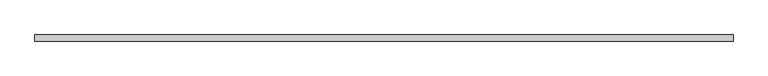
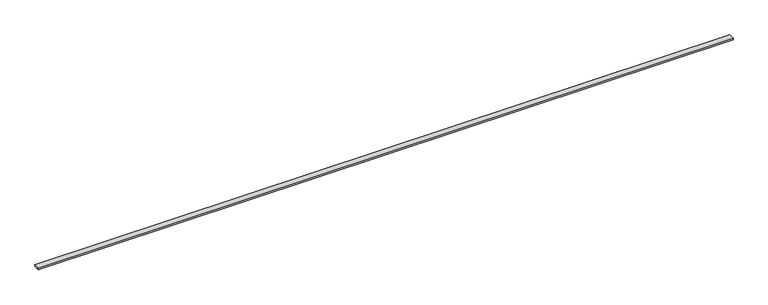
"""IFC4 building model written with IfcOpenShell, lengths in millimetres: proxy geometry, Generic Models 7:Generic Models 1:337419:Generic Models 1:337419 : Generic Models 7:Generic Models 1:337419:41 : Generic Models 7:Generic Models 1:337419:Generic Models 1:337419 : Generic Models 7:Generic Models 1:337419:301336."""

from ifc_helpers import new_model, si_unit, frame, origin, place, context, project, spatial, polyline, outline, extrude, source, transform, mapped, element, save


def generic_models_0fbd16a8(model_context):
    return source(origin(), model_context, "Body", "SweptSolid", [
        extrude(outline(polyline([(596182.8367242, -536511.1096233), (596182.8367242, -536554.1163841), (591306.0367242, -536554.1163841), (591306.0367242, -536511.1096233), (596182.8367242, -536511.1096233)])), frame((0.0, 0.0, 10085.5977062), z_axis=(0.0, 0.0, 1.0), x_axis=(1.0, 0.0, 0.0)), (0.0, 0.0, 1.0), 9.6384173),
    ])


if __name__ == "__main__":
    model = new_model("IFC4")
    model_context = context("Model", 3, world=origin())
    ifc_project = project(units=[si_unit("LENGTHUNIT", "METRE", prefix="MILLI")], contexts=[model_context])
    site = spatial("IfcSite", under=ifc_project)
    building = spatial("IfcBuilding", under=site)
    placement = place(None, origin())
    generic_models_shape = generic_models_0fbd16a8(model_context)
    element("IfcBuildingElementProxy", 1, Name="Generic Models 7:Generic Models 1:337419:Generic Models 1:337419 : Generic Models 7:Generic Models 1:337419:41 : Generic Models 7:Generic Models 1:337419:Generic Models 1:337419 : Generic Models 7:Generic Models 1:337419:301336", ObjectType="Generic Models 7:Generic Models 1:337419:Generic Models 1:337419 : Generic Models 7:Generic Models 1:337419:41 : Generic Models 7:Generic Models 1:337419:Generic Models 1:337419 : Generic Models 7:Generic Models 1:337419:301336", at=placement, inside=building, context=model_context, shape_type="MappedRepresentation", body=[
        mapped(generic_models_shape, transform((0.0, 0.0, 0.0), x_axis=(1.0, 0.0, 0.0), y_axis=(0.0, 1.0, 0.0), z_axis=(0.0, 0.0, 1.0))),
    ])
    save(model, "model.ifc")

# Revit data of these elements
# Type "Generic Models 7:Generic Models 1:337419:Generic Models 1:337419 : Generic Models 7:Generic Models 1:337419:41 : Generic Models 7:Generic Models 1:337419:Generic Models 1:337419 : Generic Models 7:Generic Models 1:337419:301336"
#   NameOverride = "Generic Models 7:Generic Models 1:337419:Generic Models 1:337419 : Generic Models 7:Generic Models 1:337419:301336"
#   ObjectTypeOverride = "Generic Models 1:337419 : Generic Models 7:Generic Models 1:337419"
#   Reference = "Generic Models 1"
#   Tag = "301336"
# Element 1 (IfcBuildingElementProxy, "Generic Models 7:Generic Models 1:337419:Generic Models 1:337419 : Generic Models 7:Generic Models 1:337419:41 : Generic Models 7:Generic Models 1:337419:Generic Models 1:337419 : Generic Models 7:Generic Models 1:337419:301336")
#   Materials on its faces: "BLOCKING - SIZE AS NEC."
# Materials
#   "BLOCKING - SIZE AS NEC.": class "Wood", colour RGB 144 113 62, transparency 0, Description = "Pinus Echinata", Cost = 0
